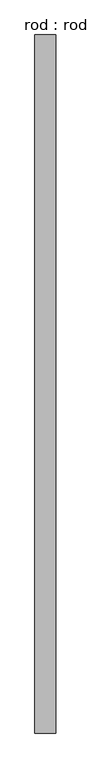
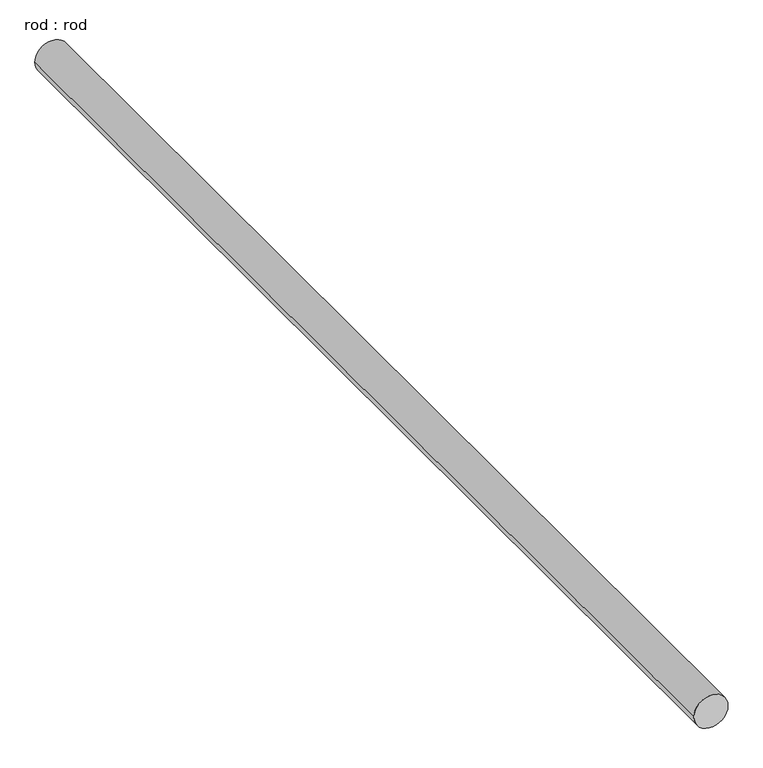
"""IFC4 building model written with IfcOpenShell, lengths in millimetres: proxy geometry, rod : rod."""

from ifc_helpers import new_model, si_unit, point, frame, frame_2d, origin, place, context, project, spatial, circle_curve, trimmed, segment, composite_curve, outline, extrude, source, transform, mapped, element, save


def rod_rod_ead96ad2(model_context):
    return source(origin(), model_context, "Body", "SweptSolid", [
        extrude(outline(composite_curve([segment(trimmed(circle_curve(frame_2d((0.0108462, 0.0)), 200.0), [point((0.0108462, 200.0))], [point((0.0108462, -200.0))], False, "CARTESIAN"), True, "CONTINUOUS"), segment(trimmed(circle_curve(frame_2d((0.0108462, 0.0)), 200.0), [point((0.0108462, -200.0))], [point((0.0108462, 200.0))], False, "CARTESIAN"), True, "CONTINUOUS")], self_intersect=False)), frame((0.0, -2592.2086565, 0.0), z_axis=(0.0, 1.0, 0.0), x_axis=(0.0, 0.0, 1.0)), (0.0, 0.0, 1.0), 13369.8745436),
    ])


if __name__ == "__main__":
    model = new_model("IFC4")
    model_context = context("Model", 3, world=origin())
    ifc_project = project(units=[si_unit("LENGTHUNIT", "METRE", prefix="MILLI")], contexts=[model_context])
    site = spatial("IfcSite", under=ifc_project)
    building = spatial("IfcBuilding", under=site)
    placement = place(None, origin())
    rod_rod_shape = rod_rod_ead96ad2(model_context)
    element("IfcBuildingElementProxy", 1, Name="rod : rod", ObjectType="rod : rod", at=placement, inside=building, context=model_context, shape_type="MappedRepresentation", body=[
        mapped(rod_rod_shape, transform((0.0, 0.0, 0.0), x_axis=(1.0, 0.0, 0.0), y_axis=(0.0, 1.0, 0.0), z_axis=(0.0, 0.0, 1.0))),
    ])
    save(model, "model.ifc")

# Revit data of these elements
# Type "rod : rod"
#   Default Elevation = 0
